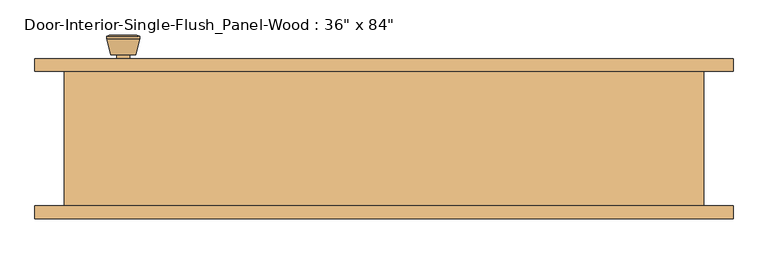
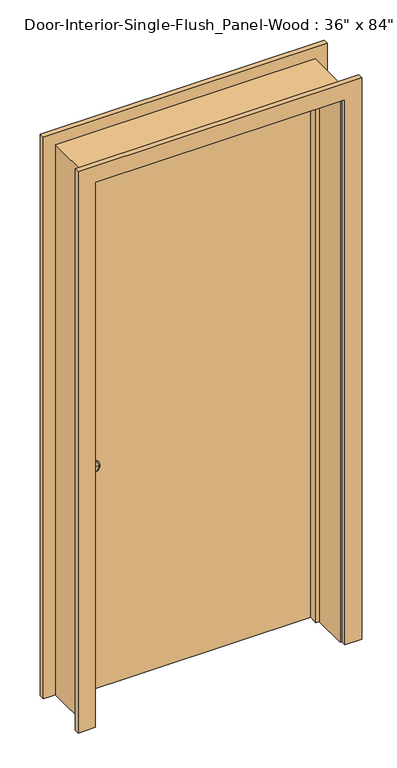
"""IFC4 building model written with IfcOpenShell, lengths in millimetres: door geometry."""

from ifc_helpers import new_model, si_unit, point, frame, frame_2d, origin, origin_with_axes, place, context, project, spatial, polyline, circle_curve, trimmed, segment, composite_curve, outline, extrude, faceted_brep, source, transform, mapped, element, save
from ifc_brep_helpers import plane_surface, cylinder_surface, revolved_surface, advanced_brep


def door_0a84c950(model_context):
    return source(origin(), model_context, "Body", "SolidModel", [
        advanced_brep(
        [(-393.7, 57.5, 914.4), (-383.7, 57.5, 914.4), (-403.7, 57.5, 914.4), (-373.2241324, 8.5, 914.4), (-393.7, 8.5, 914.4), (-414.1758676, 8.5, 914.4), (-368.7, 10.3278681, 914.4), (-418.7, 10.3278681, 914.4), (-368.7, 13.7915463, 914.4), (-418.7, 13.7915463, 914.4), (-375.063764, 38.5, 914.4), (-412.336236, 38.5, 914.4), (-383.7, 38.5, 914.4), (-403.7, 38.5, 914.4)],
        [
            (0, 1),
            (1, 2, circle_curve(frame((-393.7, 57.5, 914.4), z_axis=(0.0, 1.0, 0.0), x_axis=(-1.0, 0.0, 0.0)), 10.0)),
            (2, 0),
            (2, 1, circle_curve(frame((-393.7, 57.5, 914.4), z_axis=(0.0, 1.0, 0.0), x_axis=(-1.0, 0.0, 0.0)), 10.0)),
            (3, 4),
            (4, 5),
            (5, 3, circle_curve(frame((-393.7, 8.5, 914.4), z_axis=(0.0, -1.0, 0.0), x_axis=(-1.0, 0.0, 0.0)), 20.4758676)),
            (3, 5, circle_curve(frame((-393.7, 8.5, 914.4), z_axis=(0.0, -1.0, 0.0), x_axis=(-1.0, 0.0, 0.0)), 20.4758676)),
            (6, 3),
            (5, 7),
            (7, 6, circle_curve(frame((-393.7, 10.3278681, 914.4), z_axis=(0.0, -1.0, 0.0), x_axis=(-1.0, 0.0, 0.0)), 25.0)),
            (6, 7, circle_curve(frame((-393.7, 10.3278681, 914.4), z_axis=(0.0, -1.0, 0.0), x_axis=(-1.0, 0.0, 0.0)), 25.0)),
            (8, 6),
            (7, 9),
            (9, 8, circle_curve(frame((-393.7, 13.7915463, 914.4), z_axis=(0.0, -1.0, 0.0), x_axis=(-1.0, 0.0, 0.0)), 25.0)),
            (8, 9, circle_curve(frame((-393.7, 13.7915463, 914.4), z_axis=(0.0, -1.0, 0.0), x_axis=(-1.0, 0.0, 0.0)), 25.0)),
            (10, 8),
            (9, 11),
            (11, 10, circle_curve(frame((-393.7, 38.5, 914.4), z_axis=(0.0, -1.0, 0.0), x_axis=(-1.0, 0.0, 0.0)), 18.636236)),
            (10, 11, circle_curve(frame((-393.7, 38.5, 914.4), z_axis=(0.0, -1.0, 0.0), x_axis=(-1.0, 0.0, 0.0)), 18.636236)),
            (12, 10),
            (11, 13),
            (13, 12, circle_curve(frame((-393.7, 38.5, 914.4), z_axis=(0.0, -1.0, 0.0), x_axis=(-1.0, 0.0, 0.0)), 10.0)),
            (12, 13, circle_curve(frame((-393.7, 38.5, 914.4), z_axis=(0.0, -1.0, 0.0), x_axis=(-1.0, 0.0, 0.0)), 10.0)),
            (1, 12),
            (13, 2),
        ],
        [
            plane_surface(frame((-393.7, 57.5, 914.4), z_axis=(0.0, 1.0, 0.0), x_axis=(-1.0, 0.0, 0.0))),
            plane_surface(frame((-393.7, 8.5, 914.4), z_axis=(0.0, -1.0, 0.0), x_axis=(-1.0, 0.0, 0.0))),
            revolved_surface(polyline([(-414.1758676, 8.5, 914.4), (-418.7, 10.3278681, 914.4)]), (-393.7, 57.5, 914.4), (0.0, 1.0, 0.0)),
            cylinder_surface(frame((-393.7, 57.5, 914.4), z_axis=(0.0, 1.0, 0.0), x_axis=(-1.0, 0.0, 0.0)), 25.0),
            revolved_surface(polyline([(-418.7, 13.7915463, 914.4), (-412.336236, 38.5, 914.4)]), (-393.7, 57.5, 914.4), (0.0, 1.0, 0.0)),
            plane_surface(frame((-393.7, 38.5, 914.4), z_axis=(0.0, 1.0, 0.0), x_axis=(-1.0, 0.0, 0.0))),
            cylinder_surface(frame((-393.7, 57.5, 914.4), z_axis=(0.0, 1.0, 0.0), x_axis=(-1.0, 0.0, 0.0)), 10.0),
        ],
        [
            (0, [[1, 2, 3]]),
            (0, [[-3, 4, -1]]),
            (1, [[5, 6, 7]]),
            (1, [[-6, -5, 8]]),
            (2, [[9, -7, 10, 11]]),
            (2, [[-10, -8, -9, 12]]),
            (3, [[13, -11, 14, 15]]),
            (3, [[-14, -12, -13, 16]]),
            (4, [[17, -15, 18, 19]]),
            (4, [[-18, -16, -17, 20]]),
            (5, [[21, -19, 22, 23]]),
            (5, [[-22, -20, -21, 24]]),
            (6, [[25, -23, 26, -2]]),
            (6, [[-26, -24, -25, -4]]),
        ],
    ),
        extrude(outline(composite_curve([segment(trimmed(circle_curve(frame_2d((914.4, -393.7)), 30.0), [point((914.4, -423.7))], [point((914.4, -363.7))], False, "CARTESIAN"), True, "CONTINUOUS"), segment(trimmed(circle_curve(frame_2d((914.4, -393.7)), 30.0), [point((914.4, -363.7))], [point((914.4, -423.7))], False, "CARTESIAN"), True, "CONTINUOUS")], self_intersect=False)), frame((0.0, 57.5, 0.0), z_axis=(0.0, 1.0, 0.0), x_axis=(0.0, 0.0, 1.0)), (0.0, 0.0, 1.0), 6.0),
        advanced_brep(
        [(-393.7, 104.425, 914.4), (-403.7, 104.425, 914.4), (-383.7, 104.425, 914.4), (-373.2241324, 153.425, 914.4), (-414.1758676, 153.425, 914.4), (-393.7, 153.425, 914.4), (-368.7, 151.5971319, 914.4), (-418.7, 151.5971319, 914.4), (-368.7, 148.1334537, 914.4), (-418.7, 148.1334537, 914.4), (-375.063764, 123.425, 914.4), (-412.336236, 123.425, 914.4), (-383.7, 123.425, 914.4), (-403.7, 123.425, 914.4)],
        [
            (0, 1),
            (1, 2, circle_curve(frame((-393.7, 104.425, 914.4), z_axis=(0.0, -1.0, 0.0), x_axis=(-1.0, 0.0, 0.0)), 10.0)),
            (2, 0),
            (2, 1, circle_curve(frame((-393.7, 104.425, 914.4), z_axis=(0.0, -1.0, 0.0), x_axis=(-1.0, 0.0, 0.0)), 10.0)),
            (3, 4, circle_curve(frame((-393.7, 153.425, 914.4), z_axis=(0.0, 1.0, 0.0), x_axis=(-1.0, 0.0, 0.0)), 20.4758676)),
            (4, 5),
            (5, 3),
            (4, 3, circle_curve(frame((-393.7, 153.425, 914.4), z_axis=(0.0, 1.0, 0.0), x_axis=(-1.0, 0.0, 0.0)), 20.4758676)),
            (6, 7, circle_curve(frame((-393.7, 151.5971319, 914.4), z_axis=(0.0, 1.0, 0.0), x_axis=(-1.0, 0.0, 0.0)), 25.0)),
            (7, 4),
            (3, 6),
            (7, 6, circle_curve(frame((-393.7, 151.5971319, 914.4), z_axis=(0.0, 1.0, 0.0), x_axis=(-1.0, 0.0, 0.0)), 25.0)),
            (8, 9, circle_curve(frame((-393.7, 148.1334537, 914.4), z_axis=(0.0, 1.0, 0.0), x_axis=(-1.0, 0.0, 0.0)), 25.0)),
            (9, 7),
            (6, 8),
            (9, 8, circle_curve(frame((-393.7, 148.1334537, 914.4), z_axis=(0.0, 1.0, 0.0), x_axis=(-1.0, 0.0, 0.0)), 25.0)),
            (10, 11, circle_curve(frame((-393.7, 123.425, 914.4), z_axis=(0.0, 1.0, 0.0), x_axis=(-1.0, 0.0, 0.0)), 18.636236)),
            (11, 9),
            (8, 10),
            (11, 10, circle_curve(frame((-393.7, 123.425, 914.4), z_axis=(0.0, 1.0, 0.0), x_axis=(-1.0, 0.0, 0.0)), 18.636236)),
            (12, 13, circle_curve(frame((-393.7, 123.425, 914.4), z_axis=(0.0, 1.0, 0.0), x_axis=(-1.0, 0.0, 0.0)), 10.0)),
            (13, 11),
            (10, 12),
            (13, 12, circle_curve(frame((-393.7, 123.425, 914.4), z_axis=(0.0, 1.0, 0.0), x_axis=(-1.0, 0.0, 0.0)), 10.0)),
            (1, 13),
            (12, 2),
        ],
        [
            plane_surface(frame((-393.7, 104.425, 914.4), z_axis=(0.0, -1.0, 0.0), x_axis=(-1.0, 0.0, 0.0))),
            plane_surface(frame((-393.7, 153.425, 914.4), z_axis=(0.0, 1.0, 0.0), x_axis=(-1.0, 0.0, 0.0))),
            revolved_surface(polyline([(-414.1758676, 153.425, 914.4), (-418.7, 151.5971319, 914.4)]), (-393.7, 104.425, 914.4), (0.0, -1.0, 0.0)),
            cylinder_surface(frame((-393.7, 104.425, 914.4), z_axis=(0.0, -1.0, 0.0), x_axis=(-1.0, 0.0, 0.0)), 25.0),
            revolved_surface(polyline([(-418.7, 148.1334537, 914.4), (-412.336236, 123.425, 914.4)]), (-393.7, 104.425, 914.4), (0.0, -1.0, 0.0)),
            plane_surface(frame((-393.7, 123.425, 914.4), z_axis=(0.0, -1.0, 0.0), x_axis=(-1.0, 0.0, 0.0))),
            cylinder_surface(frame((-393.7, 104.425, 914.4), z_axis=(0.0, -1.0, 0.0), x_axis=(-1.0, 0.0, 0.0)), 10.0),
        ],
        [
            (0, [[1, 2, 3]]),
            (0, [[-3, 4, -1]]),
            (1, [[5, 6, 7]]),
            (1, [[8, -7, -6]]),
            (2, [[9, 10, -5, 11]]),
            (2, [[12, -11, -8, -10]]),
            (3, [[13, 14, -9, 15]]),
            (3, [[16, -15, -12, -14]]),
            (4, [[17, 18, -13, 19]]),
            (4, [[20, -19, -16, -18]]),
            (5, [[21, 22, -17, 23]]),
            (5, [[24, -23, -20, -22]]),
            (6, [[-2, 25, -21, 26]]),
            (6, [[-4, -26, -24, -25]]),
        ],
    ),
        extrude(outline(composite_curve([segment(trimmed(circle_curve(frame_2d((914.4, -393.7)), 30.0), [point((914.4, -423.7))], [point((914.4, -363.7))], False, "CARTESIAN"), True, "CONTINUOUS"), segment(trimmed(circle_curve(frame_2d((914.4, -393.7)), 30.0), [point((914.4, -363.7))], [point((914.4, -423.7))], False, "CARTESIAN"), True, "CONTINUOUS")], self_intersect=False)), frame((0.0, 98.425, 0.0), z_axis=(0.0, 1.0, 0.0), x_axis=(0.0, 0.0, 1.0)), (0.0, 0.0, 1.0), 6.0),
        extrude(outline(polyline([(457.2, 63.5), (-457.2, 63.5), (-457.2, 98.425), (457.2, 98.425), (457.2, 63.5)])), origin_with_axes(), (0.0, 0.0, 1.0), 2133.6),
        faceted_brep([(482.6, 98.425, 0.0), (482.6, -104.775, 0.0), (457.2, -104.775, 0.0), (457.2, 28.575, 0.0), (444.5, 28.575, 0.0), (444.5, 63.5, 0.0), (457.2, 63.5, 0.0), (457.2, 98.425, 0.0), (482.6, 98.425, 2159.0), (482.6, -104.775, 2159.0), (-482.6, -104.775, 2159.0), (-482.6, -104.775, 0.0), (-457.2, -104.775, 0.0), (-457.2, -104.775, 2133.6), (457.2, -104.775, 2133.6), (457.2, 28.575, 2133.6), (-457.2, 28.575, 2133.6), (-457.2, 28.575, 0.0), (-444.5, 28.575, 0.0), (-444.5, 28.575, 2120.9), (444.5, 28.575, 2120.9), (444.5, 63.5, 2120.9), (-444.5, 63.5, 2120.9), (-444.5, 63.5, 0.0), (-457.2, 63.5, 0.0), (-457.2, 63.5, 2133.6), (457.2, 63.5, 2133.6), (457.2, 98.425, 2133.6), (-457.2, 98.425, 2133.6), (-457.2, 98.425, 0.0), (-482.6, 98.425, 0.0), (-482.6, 98.425, 2159.0)], [[[0, 1, 2, 3, 4, 5, 6, 7]], [[1, 0, 8, 9]], [[2, 1, 9, 10, 11, 12, 13, 14]], [[3, 2, 14, 15]], [[4, 3, 15, 16, 17, 18, 19, 20]], [[5, 4, 20, 21]], [[6, 5, 21, 22, 23, 24, 25, 26]], [[7, 6, 26, 27]], [[0, 7, 27, 28, 29, 30, 31, 8]], [[9, 8, 31, 10]], [[15, 14, 13, 16]], [[21, 20, 19, 22]], [[27, 26, 25, 28]], [[30, 29, 24, 23, 18, 17, 12, 11]], [[10, 31, 30, 11]], [[16, 13, 12, 17]], [[22, 19, 18, 23]], [[28, 25, 24, 29]]]),
        extrude(outline(polyline([(0.0, 463.55), (0.0, 527.05), (2203.45, 527.05), (2203.45, -527.05), (0.0, -527.05), (0.0, -463.55), (2139.95, -463.55), (2139.95, 463.55), (0.0, 463.55)])), frame((0.0, -123.825, 0.0), z_axis=(0.0, 1.0, 0.0), x_axis=(0.0, 0.0, 1.0)), (0.0, 0.0, 1.0), 19.05),
        extrude(outline(polyline([(0.0, 463.55), (0.0, 527.05), (2203.45, 527.05), (2203.45, -527.05), (0.0, -527.05), (0.0, -463.55), (2139.95, -463.55), (2139.95, 463.55), (0.0, 463.55)])), frame((0.0, 98.425, 0.0), z_axis=(0.0, 1.0, 0.0), x_axis=(0.0, 0.0, 1.0)), (0.0, 0.0, 1.0), 19.05),
    ])


if __name__ == "__main__":
    model = new_model("IFC4")
    model_context = context("Model", 3, world=origin())
    ifc_project = project(units=[si_unit("LENGTHUNIT", "METRE", prefix="MILLI")], contexts=[model_context])
    site = spatial("IfcSite", under=ifc_project)
    building = spatial("IfcBuilding", under=site)
    placement = place(None, origin())
    door_shape = door_0a84c950(model_context)
    element("IfcDoor", 1, ObjectType="Door-Interior-Single-Flush_Panel-Wood : 36\" x 84\"", at=placement, inside=building, context=model_context, shape_type="MappedRepresentation", body=[
        mapped(door_shape, transform((0.0, 0.0, 0.0), x_axis=(1.0, 0.0, 0.0), y_axis=(0.0, 1.0, 0.0), z_axis=(0.0, 0.0, 1.0))),
    ])
    save(model, "model.ifc")

# Revit data of these elements
# Type "Door-Interior-Single-Flush_Panel-Wood : 36\" x 84\""
#   Type Mark = "1"
#   Assembly Code = "C1020300"
#   Analytic Construction = "Wooden"
#   Thickness = 0.114583 ft
#   Thermal Resistance (R) = 2.5876 (h·ft²·°F)/BTU
#   Swing Angle [instance default] = 90.00°
#   Rough Width = 3.166667 ft
#   Rough Height = 7.083333 ft
#   Height = 7.00 ft
#   Width = 3.00 ft
#   Heat Transfer Coefficient (U) = 0.3865 BTU/(h·ft²·°F)
#   Trim Material = Maple - Semigloss
#   Panel Material = Maple - Semigloss
#   Frame Material = Maple - Semigloss
#   Door Handle Material = Aluminum
#   Visual Light Transmittance = 0
#   Solar Heat Gain Coefficient = 0
#   Wall Closure = (empty or 0)
#   Function = (empty or 0)
# Element 1 (IfcDoor, "Door-Interior-Single-Flush_Panel-Wood : 36\" x 84\"")
#   Materials on its faces: "Maple - Semigloss", "Aluminum"
# Materials
#   "Maple - Semigloss": class "Wood", colour RGB 196 161 118, transparency 0, Description = "Acer Saccharum", Cost = 0
#   "Aluminum": class "Metal", colour RGB 244 245 246, transparency 0, Description = "Aluminum 6061", Cost = 0
